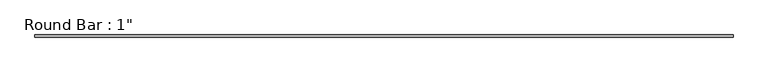
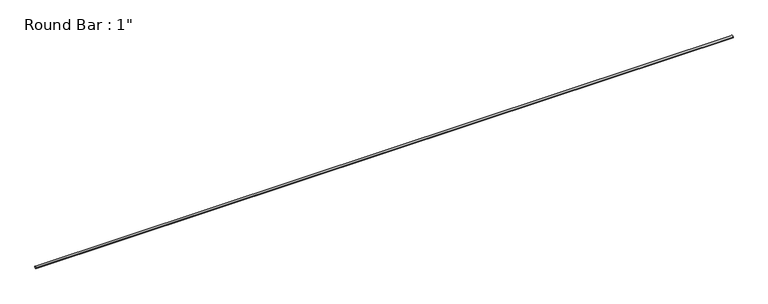
"""IFC4 building model written with IfcOpenShell, lengths in millimetres: member geometry."""

from ifc_helpers import new_model, si_unit, point, frame, origin, origin_2d, place, context, project, spatial, circle_curve, trimmed, segment, composite_curve, outline, extrude, source, transform, mapped, element, save


def member_83c2dc98(model_context):
    return source(origin(), model_context, "Body", "SweptSolid", [
        extrude(outline(composite_curve([segment(trimmed(circle_curve(origin_2d(), 12.7), [point((-12.7, 0.0))], [point((12.7, 0.0))], False, "CARTESIAN"), True, "CONTINUOUS"), segment(trimmed(circle_curve(origin_2d(), 12.7), [point((12.7, 0.0))], [point((-12.7, 0.0))], False, "CARTESIAN"), True, "CONTINUOUS")], self_intersect=False)), frame((-4095.75, 0.0, 0.0), z_axis=(1.0, 0.0, 0.0), x_axis=(0.0, 1.0, 0.0)), (0.0, 0.0, 1.0), 8191.5),
    ])


if __name__ == "__main__":
    model = new_model("IFC4")
    model_context = context("Model", 3, world=origin())
    ifc_project = project(units=[si_unit("LENGTHUNIT", "METRE", prefix="MILLI")], contexts=[model_context])
    site = spatial("IfcSite", under=ifc_project)
    building = spatial("IfcBuilding", under=site)
    placement = place(None, origin())
    member_shape = member_83c2dc98(model_context)
    element("IfcMember", 1, ObjectType="Round Bar : 1\"", at=placement, inside=building, context=model_context, shape_type="MappedRepresentation", body=[
        mapped(member_shape, transform((0.0, 0.0, 0.0), x_axis=(1.0, 0.0, 0.0), y_axis=(0.0, 1.0, 0.0), z_axis=(0.0, 0.0, 1.0))),
    ])
    save(model, "model.ifc")

# Revit data of these elements
# Type "Round Bar : 1\""
#   Assembly Code = "B10"
#   W = 0
#   Start Extension Calculation [instance default] = 10' - 0"
#   Start Extension [instance default] = -0' - 0 1/2"
#   End Extension Calculation [instance default] = 10' - 0"
#   End Extension [instance default] = -0' - 0 1/2"
#   Length [instance default] = 5' - 0"
#   d = 0' - 1"
#   A = 0 SF
#   Structural Material [instance default] = Metal - Steel - ASTM A36
# Element 1 (IfcMember, "Round Bar : 1\"")
#   Materials on its faces: "Metal - Steel - ASTM A36"
# Materials
#   "Metal - Steel - ASTM A36": class "Metal", colour RGB 199 199 199, transparency 0
